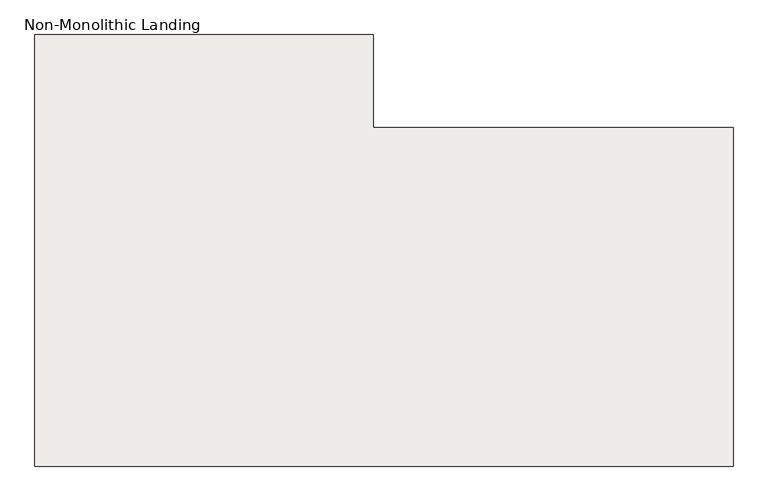
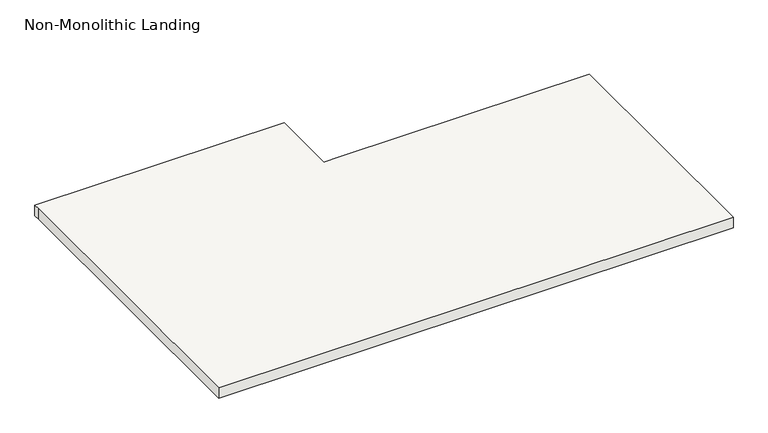
"""IFC4 building model written with IfcOpenShell, lengths in millimetres: slab geometry, Non-Monolithic Landing."""

from ifc_helpers import new_model, si_unit, frame, origin, place, context, project, spatial, polyline, outline, extrude, source, transform, mapped, element, save


def non_monolithic_landing_7c6f6286(model_context):
    return source(origin(), model_context, "Body", "SweptSolid", [
        extrude(outline(polyline([(-54750.7723171, 248286.149125), (-54750.7723171, 247270.149125), (-56846.2723171, 247270.149125), (-56846.2723171, 248540.149125), (-56846.2723171, 248565.549125), (-55830.2723171, 248565.549125), (-55830.2723171, 248540.149125), (-55830.2723171, 248286.149125), (-55766.7723171, 248286.149125), (-54750.7723171, 248286.149125)])), frame((0.0, 0.0, 1327.15), z_axis=(0.0, 0.0, 1.0), x_axis=(1.0, 0.0, 0.0)), (0.0, 0.0, 1.0), 44.45),
    ])


if __name__ == "__main__":
    model = new_model("IFC4")
    model_context = context("Model", 3, world=origin())
    ifc_project = project(units=[si_unit("LENGTHUNIT", "METRE", prefix="MILLI")], contexts=[model_context])
    site = spatial("IfcSite", under=ifc_project)
    building = spatial("IfcBuilding", under=site)
    placement = place(None, origin())
    non_monolithic_landing_shape = non_monolithic_landing_7c6f6286(model_context)
    element("IfcSlab", 1, ObjectType="Non-Monolithic Landing", at=placement, inside=building, context=model_context, shape_type="MappedRepresentation", body=[
        mapped(non_monolithic_landing_shape, transform((0.0, 0.0, 0.0), x_axis=(1.0, 0.0, 0.0), y_axis=(0.0, 1.0, 0.0), z_axis=(0.0, 0.0, 1.0))),
    ])
    save(model, "model.ifc")

# Revit data of these elements
# Element 1 (IfcSlab, "Non-Monolithic Landing")
#   Materials on its faces: "Wood - Flooring"
# Materials
#   "Wood - Flooring": class "Unassigned", colour RGB 216 169 114, transparency 0
